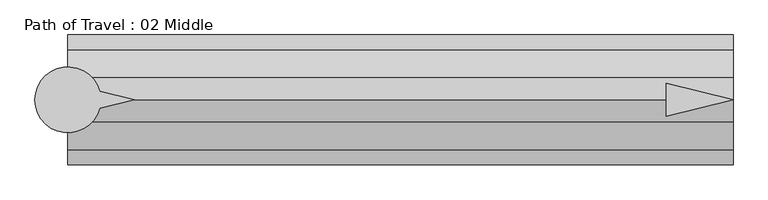
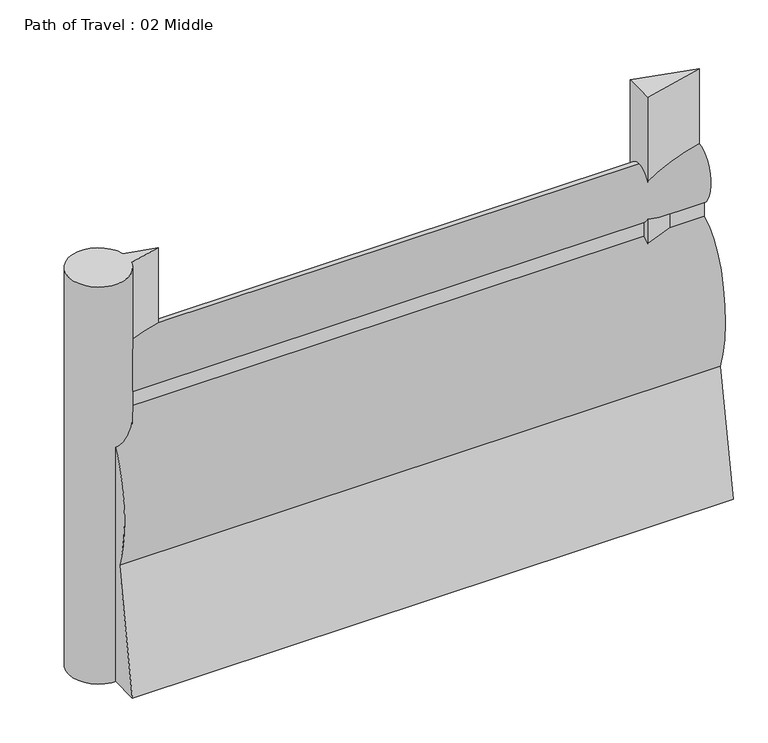
"""IFC4 building model written with IfcOpenShell, lengths in millimetres: proxy geometry, Path of Travel : 02 Middle."""

from ifc_helpers import new_model, si_unit, point, frame, frame_2d, origin, origin_with_axes, place, context, project, spatial, polyline, circle_curve, ellipse_curve, trimmed, segment, composite_curve, outline, extrude, source, transform, mapped, element, save
from ifc_brep_helpers import plane_surface, extruded_surface, advanced_brep


def path_of_travel_02_middle_d5dfa4f0(model_context):
    return source(origin(), model_context, "Body", "SolidModel", [
        advanced_brep(
        [(227.5554837, 0.0, 1727.2), (227.5554837, 42.9018657, 1436.6534209), (227.5554837, 42.9018657, 1363.4763406), (227.5554837, 184.1186263, 643.4144547), (227.5554837, 297.5699544, 0.0), (227.5554837, 145.6574193, 0.0), (227.5554837, 0.0, 584.2), (227.5554837, -145.6574193, 0.0), (227.5554837, -297.5699544, 0.0), (227.5554837, -184.1186263, 643.4144547), (227.5554837, -42.9018657, 1363.4763406), (227.5554837, -42.9018657, 1436.6534209), (3275.5554837, 0.0, 1727.2), (3275.5554837, -42.9018657, 1436.6534209), (3275.5554837, -42.9018657, 1363.4763406), (3275.5554837, -184.1186263, 643.4144547), (3275.5554837, -297.5699544, 0.0), (3275.5554837, -145.6574193, 0.0), (3275.5554837, 0.0, 584.2), (3275.5554837, 145.6574193, 0.0), (3275.5554837, 297.5699544, 0.0), (3275.5554837, 184.1186263, 643.4144547), (3275.5554837, 42.9018657, 1363.4763406), (3275.5554837, 42.9018657, 1436.6534209)],
        [
            (0, 1, ellipse_curve(frame((227.5554837, 0.0, 1574.8), z_axis=(-1.0, 0.0, 0.0), x_axis=(0.0, 0.0, 1.0)), 152.4, 101.6)),
            (1, 2),
            (2, 3, ellipse_curve(frame((227.5554837, 0.0, 914.4), z_axis=(-1.0, 0.0, 0.0), x_axis=(0.0, 0.0, -1.0)), 457.2, 228.6)),
            (3, 4),
            (4, 5),
            (5, 6),
            (6, 7),
            (7, 8),
            (8, 9),
            (9, 10, ellipse_curve(frame((227.5554837, 0.0, 914.4), z_axis=(-1.0, 0.0, 0.0), x_axis=(0.0, 0.0, -1.0)), 457.2, 228.6)),
            (10, 11),
            (11, 0, ellipse_curve(frame((227.5554837, 0.0, 1574.8), z_axis=(-1.0, 0.0, 0.0), x_axis=(0.0, 0.0, 1.0)), 152.4, 101.6)),
            (12, 13, ellipse_curve(frame((3275.5554837, 0.0, 1574.8), z_axis=(1.0, 0.0, 0.0), x_axis=(0.0, 0.0, 1.0)), 152.4, 101.6)),
            (13, 14),
            (14, 15, ellipse_curve(frame((3275.5554837, 0.0, 914.4), z_axis=(1.0, 0.0, 0.0), x_axis=(0.0, 0.0, -1.0)), 457.2, 228.6)),
            (15, 16),
            (16, 17),
            (17, 18),
            (18, 19),
            (19, 20),
            (20, 21),
            (21, 22, ellipse_curve(frame((3275.5554837, 0.0, 914.4), z_axis=(1.0, 0.0, 0.0), x_axis=(0.0, 0.0, -1.0)), 457.2, 228.6)),
            (22, 23),
            (23, 12, ellipse_curve(frame((3275.5554837, 0.0, 1574.8), z_axis=(1.0, 0.0, 0.0), x_axis=(0.0, 0.0, 1.0)), 152.4, 101.6)),
            (0, 12),
            (23, 1),
            (22, 2),
            (21, 3),
            (20, 4),
            (19, 5),
            (18, 6),
            (17, 7),
            (16, 8),
            (15, 9),
            (14, 10),
            (13, 11),
        ],
        [
            plane_surface(frame((227.5554837, 0.0, 0.0), z_axis=(-1.0, 0.0, 0.0), x_axis=(0.0, 0.0, 1.0))),
            plane_surface(frame((3275.5554837, 0.0, 0.0), z_axis=(1.0, 0.0, 0.0), x_axis=(0.0, 0.0, 1.0))),
            extruded_surface(trimmed(ellipse_curve(frame((3275.5554837, 0.0, 1574.8), z_axis=(-1.0, 0.0, 0.0), x_axis=(0.0, 0.0, 1.0)), 152.4, 101.6), [point((3275.5554837, 0.0, 1727.2))], [point((3275.5554837, 42.9018657, 1436.6534209))], True, "CARTESIAN"), (-3048.0, 0.0, 0.0), 3048.0),
            plane_surface(frame((227.5554837, 42.9018657, 1436.6534209), z_axis=(0.0, 1.0, 0.0), x_axis=(1.0, 0.0, 0.0))),
            extruded_surface(trimmed(ellipse_curve(frame((3275.5554837, 0.0, 914.4), z_axis=(-1.0, 0.0, 0.0), x_axis=(0.0, 0.0, -1.0)), 457.2, 228.6), [point((3275.5554837, 42.9018657, 1363.4763406))], [point((3275.5554837, 184.1186263, 643.4144547))], True, "CARTESIAN"), (-3048.0, 0.0, 0.0), 3048.0),
            plane_surface(frame((227.5554837, 184.1186263, 643.4144547), z_axis=(0.0, 0.9848077530122078, 0.1736481776669322), x_axis=(1.0, 0.0, 0.0))),
            plane_surface(frame((227.5554837, 297.5699544, 0.0), z_axis=(0.0, 0.0, -1.0), x_axis=(1.0, 0.0, 0.0))),
            plane_surface(frame((227.5554837, 145.6574193, 0.0), z_axis=(0.0, -0.9702957262760199, -0.2419218955995739), x_axis=(1.0, 0.0, 0.0))),
            plane_surface(frame((227.5554837, 0.0, 584.2), z_axis=(0.0, 0.9702957262759961, -0.24192189559966923), x_axis=(1.0, 0.0, 0.0))),
            plane_surface(frame((227.5554837, -145.6574193, 0.0), z_axis=(0.0, 0.0, -1.0), x_axis=(1.0, 0.0, 0.0))),
            plane_surface(frame((227.5554837, -297.5699544, 0.0), z_axis=(0.0, -0.984807753012208, 0.17364817766693066), x_axis=(1.0, 0.0, 0.0))),
            extruded_surface(trimmed(ellipse_curve(frame((3275.5554837, 0.0, 914.4), z_axis=(-1.0, 0.0, 0.0), x_axis=(0.0, 0.0, -1.0)), 457.2, 228.6), [point((3275.5554837, -184.1186263, 643.4144547))], [point((3275.5554837, -42.9018657, 1363.4763406))], True, "CARTESIAN"), (-3048.0, 0.0, 0.0), 3048.0),
            plane_surface(frame((227.5554837, -42.9018657, 1363.4763406), z_axis=(0.0, -1.0, 0.0), x_axis=(1.0, 0.0, 0.0))),
            extruded_surface(trimmed(ellipse_curve(frame((3275.5554837, 0.0, 1574.8), z_axis=(-1.0, 0.0, 0.0), x_axis=(0.0, 0.0, 1.0)), 152.4, 101.6), [point((3275.5554837, -42.9018657, 1436.6534209))], [point((3275.5554837, 0.0, 1727.2))], True, "CARTESIAN"), (-3048.0, 0.0, 0.0), 3048.0),
        ],
        [
            (0, [[1, 2, 3, 4, 5, 6, 7, 8, 9, 10, 11, 12]]),
            (1, [[13, 14, 15, 16, 17, 18, 19, 20, 21, 22, 23, 24]]),
            (2, [[-1, 25, -24, 26]]),
            (3, [[-2, -26, -23, 27]]),
            (4, [[-3, -27, -22, 28]]),
            (5, [[-4, -28, -21, 29]]),
            (6, [[-5, -29, -20, 30]]),
            (7, [[-6, -30, -19, 31]]),
            (8, [[-7, -31, -18, 32]]),
            (9, [[-8, -32, -17, 33]]),
            (10, [[-9, -33, -16, 34]]),
            (11, [[-10, -34, -15, 35]]),
            (12, [[-11, -35, -14, 36]]),
            (13, [[-12, -36, -13, -25]]),
        ],
    ),
        extrude(outline(polyline([(2969.5503371, 76.2006338), (3275.5554837, 0.0), (2969.5503371, -76.2006338), (2969.5503371, 76.2006338)])), origin_with_axes(), (0.0, 0.0, 1.0), 2129.5973753),
        extrude(outline(composite_curve([segment(polyline([(372.7837828, 39.4440225), (531.182385, 0.0), (372.7837828, -39.4440225)]), True, "CONTINUOUS"), segment(trimmed(circle_curve(frame_2d((227.2200886, 0.0)), 150.8131956), [point((372.7837828, -39.4440225))], [point((372.7837828, 39.4440225))], False, "CARTESIAN"), True, "CONTINUOUS")], self_intersect=False)), origin_with_axes(), (0.0, 0.0, 1.0), 2129.5973753),
    ])


if __name__ == "__main__":
    model = new_model("IFC4")
    model_context = context("Model", 3, world=origin())
    ifc_project = project(units=[si_unit("LENGTHUNIT", "METRE", prefix="MILLI")], contexts=[model_context])
    site = spatial("IfcSite", under=ifc_project)
    building = spatial("IfcBuilding", under=site)
    placement = place(None, origin())
    path_of_travel_02_middle_shape = path_of_travel_02_middle_d5dfa4f0(model_context)
    element("IfcBuildingElementProxy", 1, Name="Path of Travel : 02 Middle", ObjectType="Path of Travel : 02 Middle", at=placement, inside=building, context=model_context, shape_type="MappedRepresentation", body=[
        mapped(path_of_travel_02_middle_shape, transform((0.0, 0.0, 0.0), x_axis=(1.0, 0.0, 0.0), y_axis=(0.0, 1.0, 0.0), z_axis=(0.0, 0.0, 1.0))),
    ])
    save(model, "model.ifc")

# Revit data of these elements
# Type "Path of Travel : 02 Middle"
#   Path of Egress [instance default] = 4' - 0"
#   built-in parameter 1001306 [instance default] = 4 (stored number, unit not read)
#   Dot at Start = no
#   Arrow in Middle = yes
#   Arrow at End = no
#   Egress Path = none
# Element 1 (IfcBuildingElementProxy, "Path of Travel : 02 Middle")
#   Path of Egress = 10' - 0"
#   built-in parameter 1001306 = 10 (stored number, unit not read)
